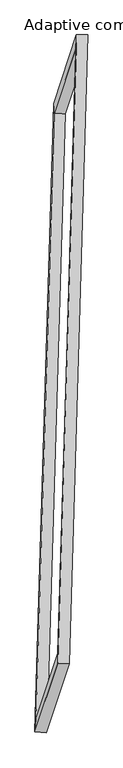
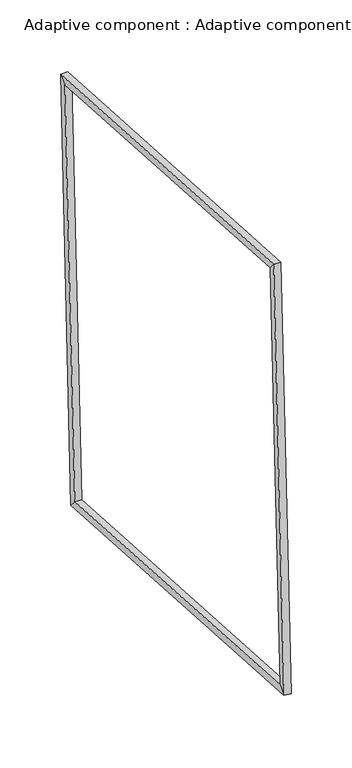
"""IFC4 building model written with IfcOpenShell, lengths in millimetres: proxy geometry, Adaptive component : Adaptive component."""

from ifc_helpers import new_model, si_unit, origin, place, context, project, spatial, faceted_brep, source, transform, mapped, element, save


def adaptive_component_adaptive_component_f098f605(model_context):
    return source(origin(), model_context, "Body", "Brep", [
        faceted_brep([(97.3329328, 1582.29231, 3137.6063486), (162.3574671, 1582.1493998, 3137.29293), (31.3649949, 1188.5947281, -812.2247374), (-33.5395398, 1189.098166, -808.2932435), (95.0786598, 1511.1740311, 3079.4359099), (-31.5074037, 1130.8580036, -737.2253521), (160.1031941, 1511.0311208, 3079.1224913), (33.3971309, 1130.3545656, -741.156846), (-76.4614533, -2424.8605356, -448.5811804), (-141.2580231, -2420.739002, -445.0137971), (-135.3693598, -2349.7401077, -386.9520029), (-70.5727901, -2353.8616413, -390.5193862), (54.5310189, -2031.3058639, 3500.936487), (-10.3855505, -2027.544858, 3500.885795), (-8.7832963, -1969.4240802, 3429.7092591), (56.133273, -1973.1850861, 3429.7599511)], [[[0, 1, 2, 3]], [[4, 0, 3, 5]], [[6, 4, 5, 7]], [[1, 6, 7, 2]], [[3, 2, 8, 9]], [[5, 3, 9, 10]], [[7, 5, 10, 11]], [[2, 7, 11, 8]], [[9, 8, 12, 13]], [[10, 9, 13, 14]], [[11, 10, 14, 15]], [[8, 11, 15, 12]], [[13, 12, 1, 0]], [[14, 13, 0, 4]], [[15, 14, 4, 6]], [[12, 15, 6, 1]]]),
    ])


if __name__ == "__main__":
    model = new_model("IFC4")
    model_context = context("Model", 3, world=origin())
    ifc_project = project(units=[si_unit("LENGTHUNIT", "METRE", prefix="MILLI")], contexts=[model_context])
    site = spatial("IfcSite", under=ifc_project)
    building = spatial("IfcBuilding", under=site)
    placement = place(None, origin())
    adaptive_component_adaptive_component_shape = adaptive_component_adaptive_component_f098f605(model_context)
    element("IfcBuildingElementProxy", 1, Name="Adaptive component : Adaptive component", ObjectType="Adaptive component : Adaptive component", at=placement, inside=building, context=model_context, shape_type="MappedRepresentation", body=[
        mapped(adaptive_component_adaptive_component_shape, transform((0.0, 0.0, 0.0), x_axis=(1.0, 0.0, 0.0), y_axis=(0.0, 1.0, 0.0), z_axis=(0.0, 0.0, 1.0))),
    ])
    save(model, "model.ifc")

# Revit data of these elements
# Type "Adaptive component : Adaptive component"
#   r [instance default] = 2063.125 mm
#   2r [instance default] = 4126.251 mm
#   Number [instance default] = 5
#   Default Elevation = 0
# Element 1 (IfcBuildingElementProxy, "Adaptive component : Adaptive component")
#   r = 2597.1 mm
#   2r = 5194.2 mm
#   Number = 24
